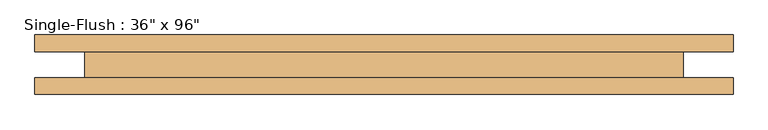
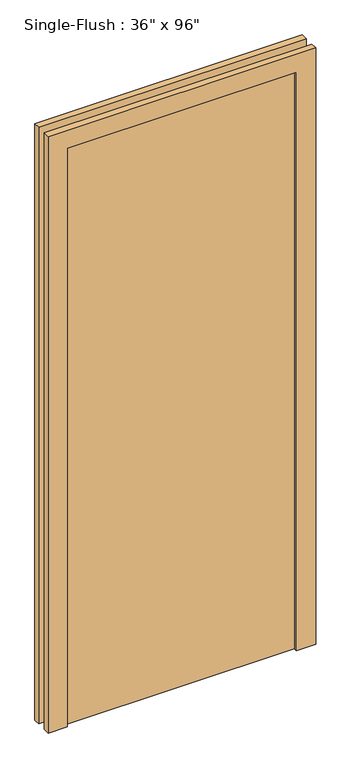
"""IFC4 building model written with IfcOpenShell, lengths in millimetres: door geometry."""

from ifc_helpers import new_model, si_unit, frame, origin, origin_with_axes, place, context, project, spatial, polyline, outline, extrude, source, transform, mapped, element, save


def door_db59b686(model_context):
    return source(origin(), model_context, "Body", "SweptSolid", [
        extrude(outline(polyline([(2514.6, -533.4), (0.0, -533.4), (0.0, -457.2), (2438.4, -457.2), (2438.4, 457.2), (0.0, 457.2), (0.0, 533.4), (2514.6, 533.4), (2514.6, -533.4)])), frame((0.0, 19.99996, 0.0), z_axis=(0.0, 1.0, 0.0), x_axis=(0.0, 0.0, 1.0)), (0.0, 0.0, 1.0), 25.4),
        extrude(outline(polyline([(2514.6, 533.4), (2514.6, -533.4), (0.0, -533.4), (0.0, -457.2), (2438.4, -457.2), (2438.4, 457.2), (0.0, 457.2), (0.0, 533.4), (2514.6, 533.4)])), frame((0.0, -45.39996, 0.0), z_axis=(0.0, 1.0, 0.0), x_axis=(0.0, 0.0, 1.0)), (0.0, 0.0, 1.0), 25.4),
        extrude(outline(polyline([(457.2, -30.80004), (-457.2, -30.80004), (-457.2, 19.99996), (457.2, 19.99996), (457.2, -30.80004)])), origin_with_axes(), (0.0, 0.0, 1.0), 2438.4),
    ])


if __name__ == "__main__":
    model = new_model("IFC4")
    model_context = context("Model", 3, world=origin())
    ifc_project = project(units=[si_unit("LENGTHUNIT", "METRE", prefix="MILLI")], contexts=[model_context])
    site = spatial("IfcSite", under=ifc_project)
    building = spatial("IfcBuilding", under=site)
    placement = place(None, origin())
    door_shape = door_db59b686(model_context)
    element("IfcDoor", 1, ObjectType="Single-Flush : 36\" x 96\"", at=placement, inside=building, context=model_context, shape_type="MappedRepresentation", body=[
        mapped(door_shape, transform((0.0, 0.0, 0.0), x_axis=(1.0, 0.0, 0.0), y_axis=(0.0, 1.0, 0.0), z_axis=(0.0, 0.0, 1.0))),
    ])
    save(model, "model.ifc")

# Revit data of these elements
# Type "Single-Flush : 36\" x 96\""
#   Type Mark = "32"
#   Construction Type Id = "MDOOR"
#   Assembly Code = "C1020"
#   Analytic Construction = "Metal"
#   Thickness = 0' - 2"
#   Heat Transfer Coefficient (U) = 3.7021 W/(m²·K)
#   Height = 8' - 0"
#   Trim Projection Ext = 0' - 1"
#   Trim Projection Int = 0' - 1"
#   Trim Width = 0' - 3"
#   Width = 3' - 0"
#   Door Material = Aluminum
#   Frame Material = Aluminum
#   Visual Light Transmittance = 0
#   Solar Heat Gain Coefficient = 0
#   Function = (empty or 0)
#   Wall Closure = (empty or 0)
# Element 1 (IfcDoor, "Single-Flush : 36\" x 96\"")
#   Materials on its faces: "Aluminum"
# Materials
#   "Aluminum": class "Metal", colour RGB 247 247 247, transparency 0, Description = "Aluminum 6061", Cost = 0
